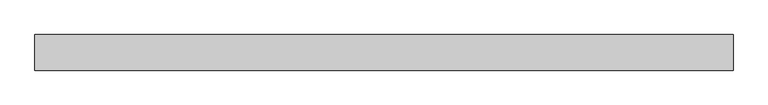
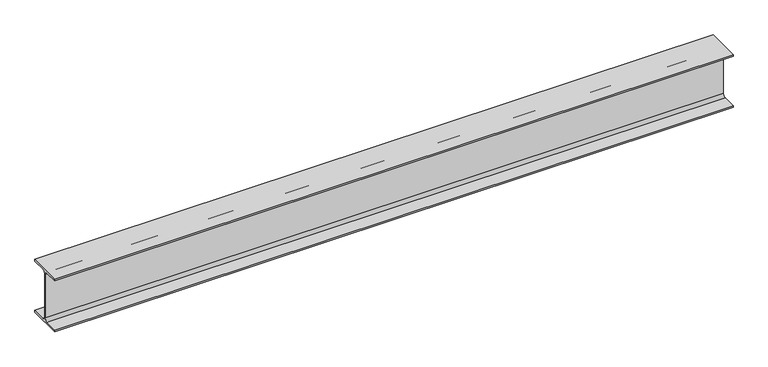
"""IFC4 building model written with IfcOpenShell, lengths in millimetres: beam geometry, 0912_Steel Framing_H-KSD3502 : H_SB_ASB_H-482x300x11x15."""

from ifc_helpers import new_model, si_unit, point, frame, frame_2d, origin, place, context, project, spatial, polyline, circle_curve, trimmed, segment, composite_curve, outline, extrude, source, transform, mapped, element, save


def beam_f3d47ea2(model_context):
    return source(origin(), model_context, "Body", "SweptSolid", [
        extrude(outline(composite_curve([segment(polyline([(150.0, -226.0), (150.0, -241.0), (-150.0, -241.0), (-150.0, -226.0), (-31.5, -226.0)]), True, "CONTINUOUS"), segment(trimmed(circle_curve(frame_2d((-31.5, -200.0)), 26.0), [point((-31.5, -226.0))], [point((-5.5, -200.0))], True, "CARTESIAN"), True, "CONTINUOUS"), segment(polyline([(-5.5, -200.0), (-5.5, 200.0)]), True, "CONTINUOUS"), segment(trimmed(circle_curve(frame_2d((-31.5, 200.0)), 26.0), [point((-5.5, 200.0))], [point((-31.5, 226.0))], True, "CARTESIAN"), True, "CONTINUOUS"), segment(polyline([(-31.5, 226.0), (-150.0, 226.0), (-150.0, 241.0), (150.0, 241.0), (150.0, 226.0), (31.5, 226.0)]), True, "CONTINUOUS"), segment(trimmed(circle_curve(frame_2d((31.5, 200.0)), 26.0), [point((31.5, 226.0))], [point((5.5, 200.0))], True, "CARTESIAN"), True, "CONTINUOUS"), segment(polyline([(5.5, 200.0), (5.5, -200.0)]), True, "CONTINUOUS"), segment(trimmed(circle_curve(frame_2d((31.5, -200.0)), 26.0), [point((5.5, -200.0))], [point((31.5, -226.0))], True, "CARTESIAN"), True, "CONTINUOUS"), segment(polyline([(31.5, -226.0), (150.0, -226.0)]), True, "CONTINUOUS")], self_intersect=False)), frame((-2939.3, 0.0, 0.0), z_axis=(1.0, 0.0, 0.0), x_axis=(0.0, 1.0, 0.0)), (0.0, 0.0, 1.0), 5878.6),
    ])


if __name__ == "__main__":
    model = new_model("IFC4")
    model_context = context("Model", 3, world=origin())
    ifc_project = project(units=[si_unit("LENGTHUNIT", "METRE", prefix="MILLI")], contexts=[model_context])
    site = spatial("IfcSite", under=ifc_project)
    building = spatial("IfcBuilding", under=site)
    placement = place(None, origin())
    beam_shape = beam_f3d47ea2(model_context)
    element("IfcBeam", 1, ObjectType="0912_Steel Framing_H-KSD3502 : H_SB_ASB_H-482x300x11x15", at=placement, inside=building, context=model_context, shape_type="MappedRepresentation", body=[
        mapped(beam_shape, transform((0.0, 0.0, 0.0), x_axis=(1.0, 0.0, 0.0), y_axis=(0.0, 1.0, 0.0), z_axis=(0.0, 0.0, 1.0))),
    ])
    save(model, "model.ifc")

# Revit data of these elements
# Type "0912_Steel Framing_H-KSD3502 : H_SB_ASB_H-482x300x11x15"
#   H_WM Code_1 = "S01AA001-00001 | Main Steel Structure Fabrication Work | Shelter/Building | Heavy Steel - Standard (Weight≥90KG/M) | Material: (   )"
#   H_WM Code_2 = "S03AA027-00001 | Main Steel Structure Erection Work | Shelter/Building | Heavy Steel (Weight≥90KG/M) | Material: (   )"
#   H_WM Code_3 = "S01AA010-00001 | Main Steel Structure Fabrication Work | Shelter/Building | Steel Painting/Coating | for Non-Fireproofed Steel Surface, Surface Preparation, Primer, Second & Final Coat | Material: (   )"
#   H_Q'ty Cal Type Tag = "SB-Q2"
#   Width = 30.0 cm
#   Web Thickness = 1.1 cm
#   Web Fillet = 2.6 cm
#   Warping Constant = 3680000.0 cm⁶
#   W = 0
#   Torsional Moment of Inertia = 88.2192 cm⁴
#   Section Area = 145.5 cm²
#   Plastic Modulus weak axis = 695.0 cm³
#   Plastic Modulus strong axis = 2790.0 cm³
#   Perimeter = 2.10 m²/m
#   Nominal Weight = 114.00 kgf/m
#   Moment of Inertia weak axis = 6760.00 cm⁴
#   Moment of Inertia strong axis = 60400.00 cm⁴
#   Height = 48.2 cm
#   Flange Thickness = 1.5 cm
#   Elastic Modulus weak axis = 451.0 cm³
#   Elastic Modulus strong axis = 2500.0 cm³
#   Centroid Vertical = 24.1 cm
#   Centroid Horizontal = 15.0 cm
#   Ix = 604000000
#   Length [instance default] = 1.5240 m
#   Zx = 2790000
#   b = 0.3000 m
#   h = 0.4820 m
#   r = 0.0260 m
#   s = 0.0110 m
#   t = 0.0150 m
#   A = 0.01455 m²
#   Structural Material [instance default] = Steel, 45-345
#   Assembly Code = ""
# Element 1 (IfcBeam, "0912_Steel Framing_H-KSD3502 : H_SB_ASB_H-482x300x11x15")
#   Structural Material = none
# Materials
#   "Steel, 45-345": class "Metal", colour RGB 189 187 185, transparency 0, Description = "Steel 345 MPa", Cost = 0
